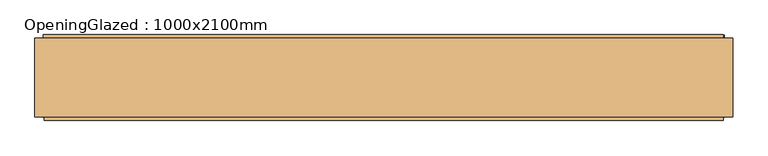
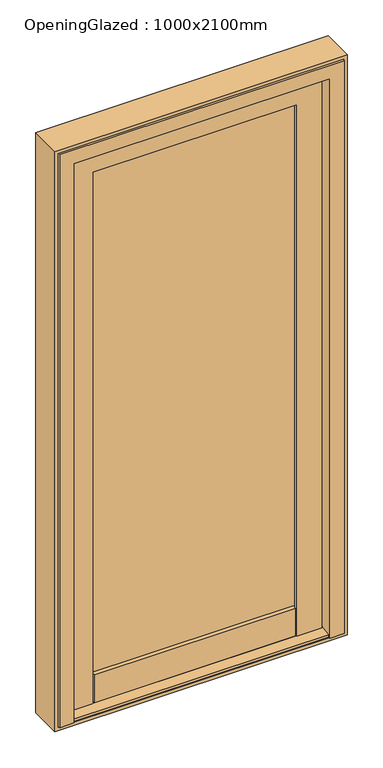
"""IFC4 building model written with IfcOpenShell, lengths in millimetres: door geometry, OpeningGlazed : 1000x2100mm."""

from ifc_helpers import new_model, si_unit, frame, origin, place, context, project, spatial, polyline, outline, extrude, faceted_brep, source, transform, mapped, element, save


def openingglazed_1000x2100mm_71b3a25b(model_context):
    return source(origin(), model_context, "Body", "SolidModel", [
        extrude(outline(polyline([(40.9999982, 133.0208766), (48.9999995, 130.8772832), (48.9999995, 112.2614733), (47.8757378, 111.1372136), (48.9999995, 110.0129457), (48.9999995, 21.4372109), (40.9999982, 21.4372109), (40.9999982, 133.0208766)])), frame((-488.0, 0.0, 0.0), z_axis=(1.0, 0.0, 0.0), x_axis=(0.0, 1.0, 0.0)), (0.0, 0.0, 1.0), 976.0),
        extrude(outline(polyline([(-16.0, 18.5055334), (50.0, 14.6999975), (50.0, 12.0), (-65.0000006, 12.0), (-65.0000006, 21.5000005), (-28.9462261, 25.9268477), (-28.000001, 28.5265826), (-16.0, 30.0000015), (-16.0, 18.5055334)])), frame((-488.0, 0.0, 0.0), z_axis=(1.0, 0.0, 0.0), x_axis=(0.0, 1.0, 0.0)), (0.0, 0.0, 1.0), 976.0),
        extrude(outline(polyline([(40.9999982, 108.2792699), (40.9999982, 15.2189343), (-16.0, 18.5055334), (-16.0, 30.0000015), (-31.0000006, 28.1582279), (-31.0000006, 129.0), (2.9999994, 133.0), (2.9999994, 112.9450831), (40.9999982, 108.2792699)])), frame((-344.5316437, 0.0, 0.0), z_axis=(1.0, 0.0, 0.0), x_axis=(0.0, 1.0, 0.0)), (0.0, 0.0, 1.0), 689.0632873),
        extrude(outline(polyline([(358.6999971, 37.9999995), (358.6999971, 33.9999989), (-358.6999971, 33.9999989), (-358.6999971, 37.9999995), (358.6999971, 37.9999995)])), frame((0.0, 0.0, 121.9447729), z_axis=(0.0, 0.0, 1.0), x_axis=(1.0, 0.0, 0.0)), (0.0, 0.0, 1.0), 1836.7552241),
        extrude(outline(polyline([(358.6999971, -15.0000005), (358.6999971, -19.0000005), (-358.6999971, -19.0000005), (-358.6999971, -15.0000005), (358.6999971, -15.0000005)])), frame((0.0, 0.0, 121.9447729), z_axis=(0.0, 0.0, 1.0), x_axis=(1.0, 0.0, 0.0)), (0.0, 0.0, 1.0), 1836.7552241),
        extrude(outline(polyline([(2100.0, 500.0), (2100.0, -500.0), (0.0, -500.0), (0.0, 500.0), (2100.0, 500.0)]), holes=[polyline([(12.0, 488.0), (12.0, -488.0), (2088.0, -488.0), (2088.0, 488.0), (12.0, 488.0)])]), frame((0.0, -68.0, 0.0), z_axis=(0.0, 1.0, 0.0), x_axis=(0.0, 0.0, 1.0)), (0.0, 0.0, 1.0), 113.0),
        faceted_brep([(486.7916962, 41.6999992, 13.2083038), (486.7916962, -73.3, 13.2083038), (437.9999993, -73.3, 13.2083038), (437.9999993, -16.0, 13.2083038), (455.8269997, -16.0, 13.2083038), (462.9116684, 41.6999992, 13.2083038), (-486.7916962, 41.6999992, 13.2083038), (-462.9116684, 41.6999992, 13.2083038), (-455.8269997, -16.0, 13.2083038), (-437.9999993, -16.0, 13.2083038), (-437.9999993, -73.3, 13.2083038), (-486.7916962, -73.3, 13.2083038), (462.9116684, 41.6999992, 2062.9116684), (-462.9116684, 41.6999992, 2062.9116684), (-486.7916962, 41.6999992, 2086.7916962), (486.7916962, 41.6999992, 2086.7916962), (486.7916962, -73.3, 2086.7916962), (-486.7916962, -73.3, 2086.7916962), (-437.9999993, -73.3, 2037.9999993), (437.9999993, -73.3, 2037.9999993), (437.9999993, -16.0, 2037.9999993), (-437.9999993, -16.0, 2037.9999993), (-455.8269997, -16.0, 2055.8269997), (455.8269997, -16.0, 2055.8269997)], [[[0, 1, 2, 3, 4, 5]], [[6, 7, 8, 9, 10, 11]], [[0, 5, 12, 13, 7, 6, 14, 15]], [[1, 0, 15, 16]], [[2, 1, 16, 17, 11, 10, 18, 19]], [[16, 15, 14, 17]], [[17, 14, 6, 11]], [[3, 2, 19, 20]], [[4, 3, 20, 21, 9, 8, 22, 23]], [[5, 4, 23, 12]], [[20, 19, 18, 21]], [[12, 23, 22, 13]], [[21, 18, 10, 9]], [[13, 22, 8, 7]]]),
        faceted_brep([(450.532936, -11.0000001, 13.2083038), (434.0000042, -11.0000001, 13.2083038), (434.0000042, -31.0000006, 13.2083038), (348.9999993, -31.0000006, 13.2083038), (345.0, 2.9999994, 13.2083038), (365.1556953, 2.9999994, 13.2083038), (369.8215082, 40.9999982, 13.2083038), (456.9177253, 40.9999982, 13.2083038), (-450.532936, -11.0000001, 13.2083038), (-456.9177253, 40.9999982, 13.2083038), (-369.8215082, 40.9999982, 13.2083038), (-365.1556953, 2.9999994, 13.2083038), (-345.0, 2.9999994, 13.2083038), (-348.9999993, -31.0000006, 13.2083038), (-434.0000042, -31.0000006, 13.2083038), (-434.0000042, -11.0000001, 13.2083038), (450.532936, -11.0000001, 2050.532936), (-450.532936, -11.0000001, 2050.532936), (-434.0000042, -11.0000001, 2034.0000042), (434.0000042, -11.0000001, 2034.0000042), (434.0000042, -31.0000006, 2034.0000042), (-434.0000042, -31.0000006, 2034.0000042), (-348.9999993, -31.0000006, 1948.9999993), (348.9999993, -31.0000006, 1948.9999993), (345.0, 2.9999994, 1945.0), (-345.0, 2.9999994, 1945.0), (-365.1556953, 2.9999994, 1965.1556953), (365.1556953, 2.9999994, 1965.1556953), (369.8215082, 40.9999982, 1969.8215082), (-369.8215082, 40.9999982, 1969.8215082), (-456.9177253, 40.9999982, 2056.9177253), (456.9177253, 40.9999982, 2056.9177253)], [[[0, 1, 2, 3, 4, 5, 6, 7]], [[8, 9, 10, 11, 12, 13, 14, 15]], [[1, 0, 16, 17, 8, 15, 18, 19]], [[2, 1, 19, 20]], [[3, 2, 20, 21, 14, 13, 22, 23]], [[4, 3, 23, 24]], [[5, 4, 24, 25, 12, 11, 26, 27]], [[6, 5, 27, 28]], [[7, 6, 28, 29, 10, 9, 30, 31]], [[0, 7, 31, 16]], [[20, 19, 18, 21]], [[24, 23, 22, 25]], [[28, 27, 26, 29]], [[16, 31, 30, 17]], [[21, 18, 15, 14]], [[25, 22, 13, 12]], [[29, 26, 11, 10]], [[17, 30, 9, 8]]]),
        faceted_brep([(486.7916962, 41.7000007, 130.8772832), (345.267467, 41.7000007, 130.8772832), (347.2234954, 48.9999995, 130.8772832), (365.8393052, 48.9999995, 130.8772832), (366.9635649, 47.8757378, 130.8772832), (368.0878328, 48.9999995, 130.8772832), (456.6635677, 48.9999995, 130.8772832), (456.6635677, 44.5786361, 130.8772832), (463.2426434, 44.5786361, 130.8772832), (463.9083032, 50.0, 130.8772832), (486.7916962, 50.0, 130.8772832), (-488.0, 41.7000007, 130.8772832), (-488.0, 50.0, 130.8772832), (-465.116607, 50.0, 130.8772832), (-464.4509472, 44.5786361, 130.8772832), (-457.8718715, 44.5786361, 130.8772832), (-457.8718715, 48.9999995, 130.8772832), (-369.2961366, 48.9999995, 130.8772832), (-368.1718687, 47.8757378, 130.8772832), (-367.047609, 48.9999995, 130.8772832), (-348.4317991, 48.9999995, 130.8772832), (-346.4757708, 41.7000007, 130.8772832), (486.7916962, 41.7000007, 2086.7916962), (-488.0, 41.7000007, 2086.7916962), (-346.4757708, 41.7000007, 1945.267467), (345.267467, 41.7000007, 1945.267467), (347.2234954, 48.9999995, 1947.2234954), (-348.4317991, 48.9999995, 1947.2234954), (-367.047609, 48.9999995, 1965.8393052), (365.8393052, 48.9999995, 1965.8393052), (366.9635649, 47.8757378, 1966.9635649), (368.0878328, 48.9999995, 1968.0878328), (-369.2961366, 48.9999995, 1968.0878328), (-457.8718715, 48.9999995, 2056.6635677), (456.6635677, 48.9999995, 2056.6635677), (456.6635677, 44.5786361, 2056.6635677), (-457.8718715, 44.5786361, 2056.6635677), (-464.4509472, 44.5786361, 2063.2426434), (463.2426434, 44.5786361, 2063.2426434), (463.9083032, 50.0, 2063.9083032), (-465.116607, 50.0, 2063.9083032), (-488.0, 50.0, 2086.7916962), (486.7916962, 50.0, 2086.7916962), (-368.1718687, 47.8757378, 1966.9635649)], [[[0, 1, 2, 3, 4, 5, 6, 7, 8, 9, 10]], [[11, 12, 13, 14, 15, 16, 17, 18, 19, 20, 21]], [[1, 0, 22, 23, 11, 21, 24, 25]], [[2, 1, 25, 26]], [[3, 2, 26, 27, 20, 19, 28, 29]], [[4, 3, 29, 30]], [[5, 4, 30, 31]], [[6, 5, 31, 32, 17, 16, 33, 34]], [[7, 6, 34, 35]], [[8, 7, 35, 36, 15, 14, 37, 38]], [[9, 8, 38, 39]], [[10, 9, 39, 40, 13, 12, 41, 42]], [[0, 10, 42, 22]], [[26, 25, 24, 27]], [[30, 29, 28, 43]], [[31, 30, 43, 32]], [[35, 34, 33, 36]], [[39, 38, 37, 40]], [[22, 42, 41, 23]], [[27, 24, 21, 20]], [[43, 28, 19, 18]], [[32, 43, 18, 17]], [[36, 33, 16, 15]], [[40, 37, 14, 13]], [[23, 41, 12, 11]]]),
    ])


if __name__ == "__main__":
    model = new_model("IFC4")
    model_context = context("Model", 3, world=origin())
    ifc_project = project(units=[si_unit("LENGTHUNIT", "METRE", prefix="MILLI")], contexts=[model_context])
    site = spatial("IfcSite", under=ifc_project)
    building = spatial("IfcBuilding", under=site)
    placement = place(None, origin())
    openingglazed_1000x2100mm_shape = openingglazed_1000x2100mm_71b3a25b(model_context)
    element("IfcDoor", 1, ObjectType="OpeningGlazed : 1000x2100mm", at=placement, inside=building, context=model_context, shape_type="MappedRepresentation", body=[
        mapped(openingglazed_1000x2100mm_shape, transform((0.0, 0.0, 0.0), x_axis=(1.0, 0.0, 0.0), y_axis=(0.0, 1.0, 0.0), z_axis=(0.0, 0.0, 1.0))),
    ])
    save(model, "model.ifc")

# Revit data of these elements
# Type "OpeningGlazed : 1000x2100mm"
#   Type IfcGUID = "0h6TxHQWH8MRgS1iM36W8s"
#   Assembly Code = "C1020700"
#   Type Mark = "198"
#   Classification.Uniclass.EF.Number = "EF_25_30"
#   Classification.Uniclass.EF.Description = "Doors and windows"
#   WindLoadRating = "n/a"
#   WaterTightnessRating = "n/a"
#   WarrantyStartDate [instance default] = "1900-12-31T23:59:59"
#   WarrantyGuarantorParts = "n/a"
#   WarrantyGuarantorLabor = "n/a"
#   WarrantyDurationUnit = "year"
#   WarrantyDurationParts = "n/a"
#   WarrantyDurationLabor = "n/a"
#   WarrantyDescription = "n/a"
#   Version = "1"
#   Uniclass2015Version = "Products v1.9"
#   Uniclass2015Title = "Composite doorsets"
#   Uniclass2015Code = "Pr_30_59_24_16"
#   TagNumber [instance default] = "n/a"
#   SustainabilityPerformance = "n/a"
#   Status = "UNSET"
#   Size = "1000 x 2100 mm"
#   Shape = "Rectangle"
#   SerialNumber [instance default] = "n/a"
#   SecurityRating = "n/a"
#   Revision = "n/a"
#   ReplacementCost = "n/a"
#   Reference = "n/a"
#   ProductInformation = "https://velfac.co.uk/Commercial/Windows-and-doors/velfac-ribo-alu-doors/13056,2299/glazed-door-ribo-alu-edo-outward-opening"
#   Name = "CompositeDoorsets_VelfacRiboAlu-OutwardOpeningGlazed_1000x2100mm_VelfacLtd"
#   NBSReference = "45-25-28/342"
#   NBSDescription = "Composite doorsets"
#   NBSCertification = "www.nationalbimlibrary.com/cert/g5unqkvs"
#   ModelReference = "VELFAC Ribo alu - Outward opening glazed door"
#   ModelNumber = "n/a"
#   MechanicalLoadRating = "n/a"
#   Material = "Wood/ aluminium"
#   ManufacturerURL = "www.velfac.co.uk"
#   ManufacturerName = "VELFAC LTD"
#   InstallationDate [instance default] = "1900-12-31T23:59:59"
#   IfcExportType = "DOOR"
#   IfcExportAs = "IfcDoorType"
#   HygrothermalRating = "n/a"
#   Grade = "n/a"
#   GlassColor = "n/a"
#   FireRating = "n/a"
#   Finish = "n/a"
#   FillGas = "n/a"
#   Features = "n/a"
#   ExpectedLife = "n/a"
#   DurationUnit = "year"
#   DurabilityRating = "n/a"
#   DoorNumber [instance default] = "n/a"
#   Description = "Glazed entrance door in wood/ aluminium for light to medium use"
#   Contact = "Marianne Gade: mg@velfac.dk"
#   Construction Type = "ALUMINIUM_WOOD"
#   Constituents = "n/a"
#   ComponentNumber [instance default] = "n/a"
#   Comment = "U-value is based on reference window 1230 x 1480 mm. For exact U-value please contact VELFAC"
#   Color = "n/a"
#   CodePerformance = "n/a"
#   Category = "Pr_30_59_24_16:Composite doorsets"
#   BarCode [instance default] = "n/a"
#   BIMObjectName = "Vlfc_VelfacLtd_CompositeDoorsets_VelfacRiboAlu-OutwardOpeningGlazed_1000x2100mm"
#   Author = "VELFAC LTD"
#   AssetType = "Fixed"
#   AssetIdentifier [instance default] = "n/a"
#   Analytic Construction = "<None>"
#   Manufacturer = "sales-support@velfac.co.uk"
#   AcousticRating = "n/a"
#   AccessibilityPerformance = "n/a"
#   WallClosure = 0.15 m
#   VisibleLightTransmittance = 0
#   VisibleLightReflectance = 0
#   ThermalTransmittanceWinter = 0
#   ThermalTransmittanceSummer = 0
#   ThermalTransmittance = 0
#   SolarTransmittance = 0
#   SolarReflectance = 0
#   SolarHeatGainTransmittance = 0
#   SolarAbsorption = 0
#   ShadingCoefficient = 0
#   PlacementSafetyIconPlan [instance default] = 0.3 m
#   PlacementSafetyIcon = 0.827 m
#   NominalWidth = 1 m
#   NominalLength = 0 m
#   NominalHeight = 2.1 m
#   Infiltration = 0
#   GlazingBarPlacementVertical = 0.438 m
#   Uw = 0.79
#   Ug = 0.52
#   StructuralOpeningWidth = 1 m
#   StructuralOpeningHeight = 2.1 m
#   LTg = 74
#   GlazingBarPlacementHorizontalTop = 0.6 m
#   GlazingBarPlacementHorizontalMiddle = 1.05 m
#   GlazingBarPlacementHorizontalBottom = 0.6 m
#   GlazingAreaFraction = 0
#   GlassThickness3 = 0 m
#   GlassThickness2 = 0.004 m
#   GlassThickness1 = 0.004 m
#   Gg = 53
#   FrameSetback [instance default] = 0.05 m
#   Eref = 5.6
#   DoorSwingOpening [instance default] = 0.926 m
#   DoorSwing [instance default] = 90.00°
#   Rough Width = 1 m
#   Rough Height = 2.1 m
#   Joint = 0.012 m
#   Height = 2.076 m
#   Width = 0.976 m
#   SmokeStop = no
#   SelfClosing = no
#   SafetyGlassPlanSouth [instance default] = no
#   SafetyGlassPlanNorth [instance default] = no
#   SafetyGlassElevation [instance default] = no
#   IsWired = no
#   IsTempered = no
#   IsLaminated = no
#   IsExternal = yes
#   IsCoated = no
#   HasGlazingBar68mmHorizontalTop = no
#   HasGlazingBar68mmHorizontalBottom = no
#   HasDrive = no
#   HandicapAccessible = yes
#   SashOpeningRight [instance default] = yes
#   SashOpeningLeft [instance default] = yes
#   GlassLayers = 2
#   FrameDepth148mm = no
#   FrameDepth123mm = yes
#   FireExit = no
#   HasGlazingBar68mmVertical = no
#   HasGlazingBar31mmEnergyVertical = no
#   HasGlazingBar31mmEnergyHorizontalTop = no
#   HasGlazingBar31mmEnergyHorizontalBottom = no
#   HasGlazingBar68mmHorizontalMiddle = no
#   HasGlazingBar31mmEnergyHorizontalMiddle = no
#   ThresholdMaterial = Vlfc_VelfacLtd_Frame
#   GlazingPanelMaterial = Vlfc_VelfacLtd_Glass_Double
#   FrameMaterialInternal = Vlfc_VelfacLtd_Paint_White
#   FrameMaterialExternal = Vlfc_VelfacLtd_Frame
#   Type Comments = ""
#   Thickness = 0
#   Operation = ""
#   Keynote = ""
#   Fire Rating = ""
#   URL = ""
#   Model = ""
#   Function = (empty or 0)
#   Wall Closure = (empty or 0)
# Element 1 (IfcDoor, "OpeningGlazed : 1000x2100mm")
#   FrameSetback = 0 m
#   Materials on its faces: "Vlfc_VelfacLtd_Frame", "Vlfc_VelfacLtd_Paint_White", "Vlfc_VelfacLtd_Glass_Double"
# Materials
#   "Vlfc_VelfacLtd_Frame": class "Unassigned", colour RGB 80 80 80, transparency 0, Cost = 0
#   "Vlfc_VelfacLtd_Glass_Double": class "Glass", colour RGB 0 0 255, transparency 0.75, Cost = 0
#   "Vlfc_VelfacLtd_Paint_White": class "Paint/Coating", colour RGB 255 255 255, transparency 0, Cost = 0
